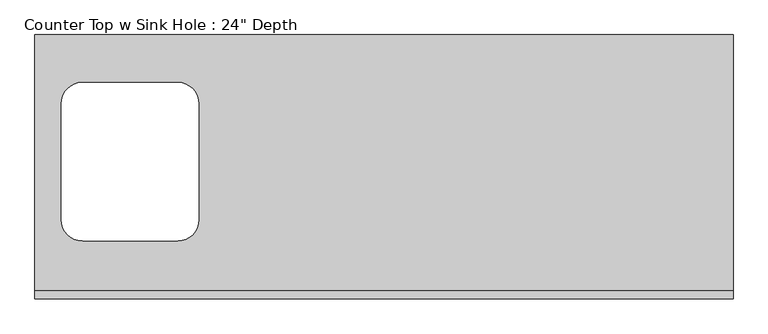
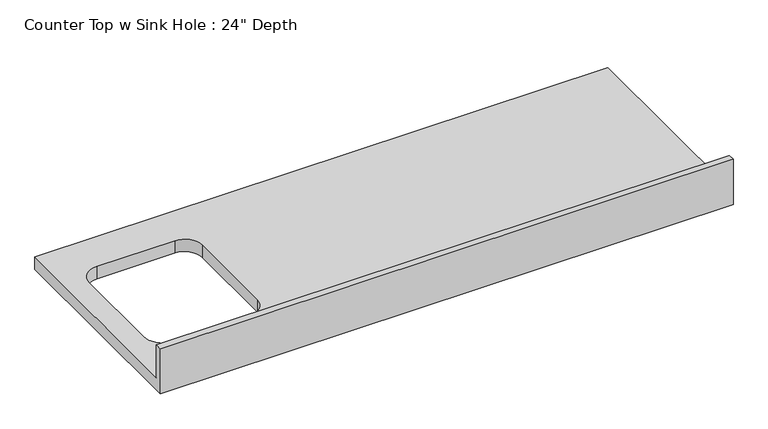
"""IFC4 building model written with IfcOpenShell, lengths in millimetres: furniture geometry."""

from ifc_helpers import new_model, si_unit, frame, origin, place, context, project, spatial, polyline, circle_curve, source, transform, mapped, element, save
from ifc_brep_helpers import plane_surface, revolved_surface, advanced_brep


def furniture_0e5e29b4(model_context):
    return source(origin(), model_context, "Body", "AdvancedBrep", [
        advanced_brep(
        [(-1200.4622951, 635.0, 914.4), (-1200.4622951, 19.05, 914.4), (475.9377049, 19.05, 914.4), (475.9377049, 635.0, 914.4), (-1086.1622951, 139.7, 914.4), (-1136.9622951, 190.5, 914.4), (-1136.9622951, 469.9, 914.4), (-1086.1622951, 520.7, 914.4), (-857.5622951, 520.7, 914.4), (-806.7622951, 469.9, 914.4), (-806.7622951, 190.5, 914.4), (-857.5622951, 139.7, 914.4), (475.9377049, 0.0, 876.3), (-1200.4622951, 0.0, 876.3), (-1200.4622951, 635.0, 876.3), (475.9377049, 635.0, 876.3), (-857.5622951, 139.7, 876.3), (-806.7622951, 190.5, 876.3), (-806.7622951, 469.9, 876.3), (-857.5622951, 520.7, 876.3), (-1086.1622951, 520.7, 876.3), (-1136.9622951, 469.9, 876.3), (-1136.9622951, 190.5, 876.3), (-1086.1622951, 139.7, 876.3), (475.9377049, 0.0, 1016.0), (-1200.4622951, 0.0, 1016.0), (-1200.4622951, 19.05, 1016.0), (475.9377049, 19.05, 1016.0)],
        [
            (0, 1),
            (1, 2),
            (2, 3),
            (3, 0),
            (4, 5, circle_curve(frame((-1086.1622951, 190.5, 914.4), z_axis=(0.0, 0.0, -1.0), x_axis=(1.0, 0.0, 0.0)), 50.8)),
            (5, 6),
            (6, 7, circle_curve(frame((-1086.1622951, 469.9, 914.4), z_axis=(0.0, 0.0, -1.0), x_axis=(1.0, 0.0, 0.0)), 50.8)),
            (7, 8),
            (8, 9, circle_curve(frame((-857.5622951, 469.9, 914.4), z_axis=(0.0, 0.0, -1.0), x_axis=(1.0, 0.0, 0.0)), 50.8)),
            (9, 10),
            (10, 11, circle_curve(frame((-857.5622951, 190.5, 914.4), z_axis=(0.0, 0.0, -1.0), x_axis=(1.0, 0.0, 0.0)), 50.8)),
            (11, 4),
            (12, 13),
            (13, 14),
            (14, 15),
            (15, 12),
            (16, 17, circle_curve(frame((-857.5622951, 190.5, 876.3), z_axis=(0.0, 0.0, 1.0), x_axis=(1.0, 0.0, 0.0)), 50.8)),
            (17, 18),
            (18, 19, circle_curve(frame((-857.5622951, 469.9, 876.3), z_axis=(0.0, 0.0, 1.0), x_axis=(1.0, 0.0, 0.0)), 50.8)),
            (19, 20),
            (20, 21, circle_curve(frame((-1086.1622951, 469.9, 876.3), z_axis=(0.0, 0.0, 1.0), x_axis=(1.0, 0.0, 0.0)), 50.8)),
            (21, 22),
            (22, 23, circle_curve(frame((-1086.1622951, 190.5, 876.3), z_axis=(0.0, 0.0, 1.0), x_axis=(1.0, 0.0, 0.0)), 50.8)),
            (23, 16),
            (12, 24),
            (24, 25),
            (25, 13),
            (25, 26),
            (26, 1),
            (0, 14),
            (3, 15),
            (2, 27),
            (27, 24),
            (11, 16),
            (23, 4),
            (22, 5),
            (21, 6),
            (20, 7),
            (19, 8),
            (18, 9),
            (17, 10),
            (27, 26),
        ],
        [
            plane_surface(frame((-1200.4622951, 0.0, 914.4), z_axis=(0.0, 0.0, 1.0), x_axis=(-1.0, 0.0, 0.0))),
            plane_surface(frame((-1200.4622951, 0.0, 876.3), z_axis=(0.0, 0.0, -1.0), x_axis=(1.0, 0.0, 0.0))),
            plane_surface(frame((475.9377049, 0.0, 914.4), z_axis=(0.0, -1.0, 0.0), x_axis=(0.0, 0.0, -1.0))),
            plane_surface(frame((-1200.4622951, 0.0, 914.4), z_axis=(-1.0, 0.0, 0.0), x_axis=(0.0, 0.0, -1.0))),
            plane_surface(frame((-1200.4622951, 635.0, 914.4), z_axis=(0.0, 1.0, 0.0), x_axis=(0.0, 0.0, -1.0))),
            plane_surface(frame((475.9377049, 635.0, 914.4), z_axis=(1.0, 0.0, 0.0), x_axis=(0.0, 0.0, -1.0))),
            plane_surface(frame((-857.5622951, 139.7, 914.4), z_axis=(0.0, 1.0, 0.0), x_axis=(0.0, 0.0, -1.0))),
            revolved_surface(polyline([(-1035.3622951, 190.5, 914.4), (-1035.3622951, 190.5, 876.3)]), (-1086.1622951, 190.5, 876.3), (0.0, 0.0, 1.0)),
            plane_surface(frame((-1136.9622951, 190.5, 914.4), z_axis=(1.0, 0.0, 0.0), x_axis=(0.0, 0.0, -1.0))),
            revolved_surface(polyline([(-1035.3622951, 469.9, 914.4), (-1035.3622951, 469.9, 876.3)]), (-1086.1622951, 469.9, 876.3), (0.0, 0.0, 1.0)),
            plane_surface(frame((-1086.1622951, 520.7, 914.4), z_axis=(0.0, -1.0, 0.0), x_axis=(0.0, 0.0, -1.0))),
            revolved_surface(polyline([(-806.7622951000001, 469.9, 914.4), (-806.7622951000001, 469.9, 876.3)]), (-857.5622951, 469.9, 876.3), (0.0, 0.0, 1.0)),
            plane_surface(frame((-806.7622951, 469.9, 914.4), z_axis=(-1.0, 0.0, 0.0), x_axis=(0.0, 0.0, -1.0))),
            revolved_surface(polyline([(-806.7622951000001, 190.5, 914.4), (-806.7622951000001, 190.5, 876.3)]), (-857.5622951, 190.5, 876.3), (0.0, 0.0, 1.0)),
            plane_surface(frame((-1200.4622951, 0.0, 1016.0), z_axis=(0.0, 0.0, 1.0), x_axis=(0.0, 1.0, 0.0))),
            plane_surface(frame((-1200.4622951, 19.05, 1016.0), z_axis=(0.0, 1.0, 0.0), x_axis=(0.0, 0.0, -1.0))),
        ],
        [
            (0, [[1, 2, 3, 4], [5, 6, 7, 8, 9, 10, 11, 12]]),
            (1, [[13, 14, 15, 16], [17, 18, 19, 20, 21, 22, 23, 24]]),
            (2, [[25, 26, 27, -13]]),
            (3, [[-27, 28, 29, -1, 30, -14]]),
            (4, [[31, -15, -30, -4]]),
            (5, [[-31, -3, 32, 33, -25, -16]]),
            (6, [[-12, 34, -24, 35]]),
            (7, [[-23, 36, -5, -35]]),
            (8, [[-22, 37, -6, -36]]),
            (9, [[-21, 38, -7, -37]]),
            (10, [[-20, 39, -8, -38]]),
            (11, [[-19, 40, -9, -39]]),
            (12, [[-18, 41, -10, -40]]),
            (13, [[-11, -41, -17, -34]]),
            (14, [[-26, -33, 42, -28]]),
            (15, [[-32, -2, -29, -42]]),
        ],
    ),
    ])


if __name__ == "__main__":
    model = new_model("IFC4")
    model_context = context("Model", 3, world=origin())
    ifc_project = project(units=[si_unit("LENGTHUNIT", "METRE", prefix="MILLI")], contexts=[model_context])
    site = spatial("IfcSite", under=ifc_project)
    building = spatial("IfcBuilding", under=site)
    placement = place(None, origin())
    furniture_shape = furniture_0e5e29b4(model_context)
    element("IfcFurniture", 1, ObjectType="Counter Top w Sink Hole : 24\" Depth", at=placement, inside=building, context=model_context, shape_type="MappedRepresentation", body=[
        mapped(furniture_shape, transform((0.0, 0.0, 0.0), x_axis=(1.0, 0.0, 0.0), y_axis=(0.0, 1.0, 0.0), z_axis=(0.0, 0.0, 1.0))),
    ])
    save(model, "model.ifc")

# Revit data of these elements
# Type "Counter Top w Sink Hole : 24\" Depth"
#   Assembly Code = "C1030400"
#   Counter Thickness = 0' - 1 1/2"
#   Depth = 2' - 1"
#   Height = 3' - 0"
#   Length [instance default] = 8' - 0"
#   Sink Location [instance default] = 2' - 0"
#   Sink Location To Wall [instance default] = 0' - 6"
#   Sink Opening Depth [instance default] = 1' - 3"
#   Sink Opening Width [instance default] = 2' - 3"
#   Counter Top Material = none
#   Default Elevation = 0
# Element 1 (IfcFurniture, "Counter Top w Sink Hole : 24\" Depth")
#   Length = 5' - 6"
#   Sink Location = 0' - 9"
#   Sink Opening Depth = 1' - 2"
#   Sink Opening Width = 1' - 0"
#   Materials on its faces: "Counter Top"
# Materials
#   "Counter Top": class "Unassigned", colour RGB 226 177 128, transparency 0
